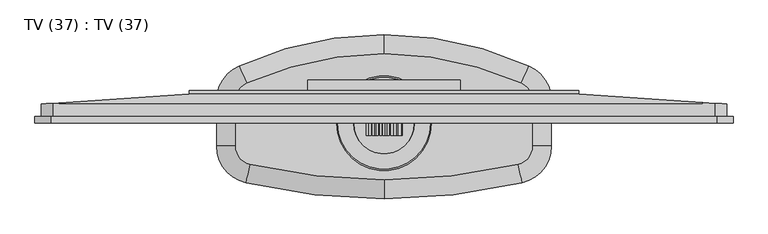
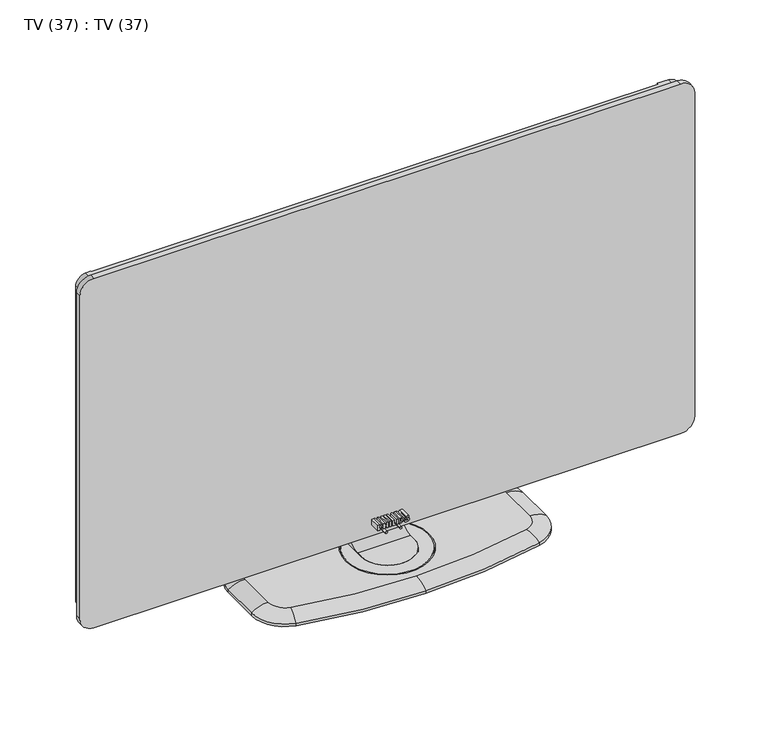
"""IFC4 building model written with IfcOpenShell, lengths in millimetres: furniture geometry, TV (37) : TV (37)."""

import ifcopenshell
import ifcopenshell.guid

model = None  # the IFC model being written
_history = None  # IfcOwnerHistory: only IFC2X3 demands one
_inside = {}  # id of a spatial element -> (the spatial element, [elements in it])
_under = {}  # id of a project, library or spatial element -> (it, [spatial elements below it])
_declared = {}  # id of a project -> (the project, [libraries it declares])
_typed = {}  # id of a type object -> (the type object, [elements of that type])
_made_of = {}  # id of a material, layer set ... -> (it, [elements and type objects made of it])


def new_model(schema):
    """Start an empty IFC model of exactly this schema.

    Asked for "IFC4X3", IfcOpenShell would pick the latest addendum, in which some entities
    have other attributes; the version numbers below select the first issue.
    IFC2X3 requires an IfcOwnerHistory on every rooted entity: one is made here for all.
    """
    global model, _history
    if schema == "IFC4X3":
        model = ifcopenshell.file(schema_version=(4, 3, 0, 0))
    else:
        model = ifcopenshell.file(schema=schema)
    _inside.clear()
    _under.clear()
    _declared.clear()
    _typed.clear()
    _made_of.clear()
    _history = None
    if model.schema == "IFC2X3":
        org = make("IfcOrganization", Name="unknown")
        user = make(
            "IfcPersonAndOrganization",
            ThePerson=make("IfcPerson", FamilyName="unknown"),
            TheOrganization=org,
        )
        app = make(
            "IfcApplication",
            ApplicationDeveloper=org,
            Version="unknown",
            ApplicationFullName="unknown",
            ApplicationIdentifier="unknown",
        )
        _history = make(
            "IfcOwnerHistory",
            OwningUser=user,
            OwningApplication=app,
            ChangeAction="ADDED",
            CreationDate=0,
        )
    return model


def make(cls, **values):
    """One entity of the class cls with the attributes given. An attribute that is None is left unset."""
    return model.create_entity(
        cls, **{name: value for name, value in values.items() if value is not None}
    )


def rooted(cls, **values):
    """An entity with a GlobalId (a new one), such as an element, a storey or a relation."""
    return make(cls, GlobalId=ifcopenshell.guid.new(), OwnerHistory=_history, **values)


def si_unit(unit_type, name, prefix=None):
    """IfcSIUnit, for example si_unit("LENGTHUNIT", "METRE", prefix="MILLI")."""
    return make("IfcSIUnit", UnitType=unit_type, Prefix=prefix, Name=name)


def assignment(units):
    """IfcUnitAssignment: the units of a project."""
    return None if units is None else make("IfcUnitAssignment", Units=units)


def point(xyz):
    """IfcCartesianPoint."""
    return None if xyz is None else make("IfcCartesianPoint", Coordinates=xyz)


def direction(xyz):
    """IfcDirection."""
    return None if xyz is None else make("IfcDirection", DirectionRatios=xyz)


def frame(location, z_axis=None, x_axis=None):
    """IfcAxis2Placement3D, a coordinate frame: its origin and axes. An axis left out is left unset."""
    return make(
        "IfcAxis2Placement3D",
        Location=point(location),
        Axis=direction(z_axis),
        RefDirection=direction(x_axis),
    )


def frame_2d(location, x_axis=None):
    """IfcAxis2Placement2D, a coordinate frame in the plane: its origin and x axis."""
    return make(
        "IfcAxis2Placement2D", Location=point(location), RefDirection=direction(x_axis)
    )


def origin():
    """The frame at (0, 0, 0) with its axes left unset."""
    return frame((0.0, 0.0, 0.0))


def place(relative_to, where):
    """IfcLocalPlacement: puts the frame where relative to a parent placement (None: the world)."""
    return make(
        "IfcLocalPlacement", PlacementRelTo=relative_to, RelativePlacement=where
    )


def context(
    kind, dimensions, precision=None, world=None, true_north=None, identifier=None
):
    """IfcGeometricRepresentationContext, for example the 3D "Model" context."""
    return make(
        "IfcGeometricRepresentationContext",
        ContextIdentifier=identifier,
        ContextType=kind,
        CoordinateSpaceDimension=dimensions,
        Precision=precision,
        WorldCoordinateSystem=world,
        TrueNorth=true_north,
    )


def project(units=None, contexts=None):
    """IfcProject with its units and contexts."""
    return rooted(
        "IfcProject",
        Name="project",
        RepresentationContexts=contexts,
        UnitsInContext=assignment(units),
    )


def spatial(cls, under=None, at=None, **own):
    """A site, building, storey or space (cls), placed at a placement, below another one or the project."""
    s = rooted(cls, ObjectPlacement=at, **own)
    if under is not None:
        _under.setdefault(under.id(), (under, []))[1].append(s)
    return s


def polyline(points):
    """IfcPolyline through the points."""
    return make("IfcPolyline", Points=[point(p) for p in points])


def circle_curve(where, radius):
    """IfcCircle in the frame where."""
    return make("IfcCircle", Position=where, Radius=radius)


def ellipse_curve(where, semi_axis1, semi_axis2):
    """IfcEllipse in the frame where."""
    return make(
        "IfcEllipse", Position=where, SemiAxis1=semi_axis1, SemiAxis2=semi_axis2
    )


def trimmed(basis, trim1, trim2, sense, master):
    """IfcTrimmedCurve: the piece of a basis curve between two trims."""
    return make(
        "IfcTrimmedCurve",
        BasisCurve=basis,
        Trim1=trim1,
        Trim2=trim2,
        SenseAgreement=sense,
        MasterRepresentation=master,
    )


def segment(curve, same_sense, transition):
    """IfcCompositeCurveSegment."""
    return make(
        "IfcCompositeCurveSegment",
        Transition=transition,
        SameSense=same_sense,
        ParentCurve=curve,
    )


def composite_curve(segments, self_intersect=None):
    """IfcCompositeCurve: segments joined end to end."""
    return make("IfcCompositeCurve", Segments=segments, SelfIntersect=self_intersect)


def outline(outer, holes=None, kind="AREA"):
    """IfcArbitraryClosedProfileDef: a profile drawn as a closed curve; with holes, ...WithVoids."""
    if holes is None:
        return make("IfcArbitraryClosedProfileDef", ProfileType=kind, OuterCurve=outer)
    return make(
        "IfcArbitraryProfileDefWithVoids",
        ProfileType=kind,
        OuterCurve=outer,
        InnerCurves=holes,
    )


def extrude(swept, where, along, depth):
    """IfcExtrudedAreaSolid: the profile swept, set in the frame where, extruded along a direction by depth."""
    return make(
        "IfcExtrudedAreaSolid",
        SweptArea=swept,
        Position=where,
        ExtrudedDirection=direction(along),
        Depth=depth,
    )


def shape(context_of_items, identifier, shape_type, items):
    """IfcShapeRepresentation: the items that make up one representation, for example the "Body"."""
    return make(
        "IfcShapeRepresentation",
        ContextOfItems=context_of_items,
        RepresentationIdentifier=identifier,
        RepresentationType=shape_type,
        Items=items,
    )


def source(mapping_origin, context_of_items, identifier, shape_type, items):
    """IfcRepresentationMap: a shape defined once, which mapped items show again and again."""
    return make(
        "IfcRepresentationMap",
        MappingOrigin=mapping_origin,
        MappedRepresentation=shape(context_of_items, identifier, shape_type, items),
    )


def transform(
    local_origin,
    x_axis=None,
    y_axis=None,
    z_axis=None,
    scale=None,
    scale2=None,
    scale3=None,
    uniform=True,
):
    """IfcCartesianTransformationOperator3D, or its non-uniform kind. x_axis, y_axis, z_axis: its Axis1, 2, 3."""
    if uniform:
        return make(
            "IfcCartesianTransformationOperator3D",
            Axis1=direction(x_axis),
            Axis2=direction(y_axis),
            LocalOrigin=point(local_origin),
            Scale=scale,
            Axis3=direction(z_axis),
        )
    return make(
        "IfcCartesianTransformationOperator3DnonUniform",
        Axis1=direction(x_axis),
        Axis2=direction(y_axis),
        LocalOrigin=point(local_origin),
        Scale=scale,
        Axis3=direction(z_axis),
        Scale2=scale2,
        Scale3=scale3,
    )


def mapped(mapping_source, mapping_target):
    """IfcMappedItem: shows the shape of a source again, moved by a transform."""
    return make(
        "IfcMappedItem", MappingSource=mapping_source, MappingTarget=mapping_target
    )


def made_of(thing, what):
    """Note that an element or type object is made of a material, layer set ...; save() writes the relation."""
    if what is not None:
        _made_of.setdefault(what.id(), (what, []))[1].append(thing)
    return thing


def element(
    cls,
    number,
    at=None,
    inside=None,
    cuts=None,
    type_object=None,
    material=None,
    context=None,
    identifier="Body",
    shape_type=None,
    held_by="IfcProductDefinitionShape",
    body=None,
    shapes=None,
    **own,
):
    """One element of the class cls, such as IfcWall. Its Tag is "e" and its number.

    at: its placement. inside: the storey or other place that contains it. cuts: it is an
    opening in that element (IfcRelVoidsElement). A single representation is given by context,
    identifier, shape_type and body (its items); several are given by shapes. held_by: the class
    of the entity that holds the representations. save() writes the other relations.
    """
    e = rooted(cls, Tag="e%d" % number, ObjectPlacement=at, **own)
    if body is not None:
        shapes = [shape(context, identifier, shape_type, body)]
    if shapes is not None:
        e.Representation = make(held_by, Representations=shapes)
    if inside is not None:
        _inside.setdefault(inside.id(), (inside, []))[1].append(e)
    if cuts is not None:
        rooted(
            "IfcRelVoidsElement", RelatingBuildingElement=cuts, RelatedOpeningElement=e
        )
    if type_object is not None:
        _typed.setdefault(type_object.id(), (type_object, []))[1].append(e)
    return made_of(e, material)


def aggregate(whole, parts):
    """IfcRelAggregates: a whole, such as a stair, and the parts it consists of."""
    return rooted("IfcRelAggregates", RelatingObject=whole, RelatedObjects=parts)


def save(model, path):
    """Write the relations noted so far, then the file.

    IfcRelAggregates (storeys below a building ...), IfcRelContainedInSpatialStructure (elements
    in a storey), IfcRelDefinesByType, IfcRelAssociatesMaterial and IfcRelDeclares: one each for
    every whole, place, type object, material and project.
    """
    for whole, parts in _under.values():
        aggregate(whole, parts)
    for where, things in _inside.values():
        rooted(
            "IfcRelContainedInSpatialStructure",
            RelatedElements=things,
            RelatingStructure=where,
        )
    for kind, things in _typed.values():
        rooted("IfcRelDefinesByType", RelatedObjects=things, RelatingType=kind)
    for what, things in _made_of.values():
        rooted("IfcRelAssociatesMaterial", RelatedObjects=things, RelatingMaterial=what)
    for by, libraries in _declared.values():
        rooted("IfcRelDeclares", RelatingContext=by, RelatedDefinitions=libraries)
    model.write(path)


def plane_surface(at):
    """IfcPlane: the flat surface through the origin of the frame at, square to its z axis."""
    return make("IfcPlane", Position=at)


def cylinder_surface(at, radius):
    """IfcCylindricalSurface: all points at the distance radius from the z axis of the frame at."""
    return make("IfcCylindricalSurface", Position=at, Radius=radius)


def revolved_surface(curve, axis_point, axis_direction):
    """IfcSurfaceOfRevolution: the curve turned about the line through axis_point along axis_direction."""
    return make(
        "IfcSurfaceOfRevolution",
        SweptCurve=make("IfcArbitraryOpenProfileDef", ProfileType="CURVE", Curve=curve),
        AxisPosition=make("IfcAxis1Placement", Location=point(axis_point), Axis=direction(axis_direction)),
    )


def advanced_brep(points, edges, surfaces, faces):
    """IfcAdvancedBrep: a solid bounded by faces that lie on surfaces and meet in shared edges.

    An edge is (start, end): straight between two places in points (the first is 0);
    or (start, end, curve); or (start, end, curve, False) where it runs against its curve.
    A face is (place in surfaces, loops), or (place, loops, False) where it looks against
    its surface's normal. A loop lists edges by number (the first is 1), with a minus sign
    where the edge is run from its end to its start. The first loop is the outer one.
    """
    corners = [point(p) for p in points]
    vertices = [make("IfcVertexPoint", VertexGeometry=c) for c in corners]
    made = []
    for start, end, *more in edges:
        made.append(
            make(
                "IfcEdgeCurve",
                EdgeStart=vertices[start],
                EdgeEnd=vertices[end],
                EdgeGeometry=more[0] if more else make("IfcPolyline", Points=[corners[start], corners[end]]),
                SameSense=more[1] if len(more) > 1 else True,
            )
        )
    hull = []
    for where, loops, *sense in faces:
        bounds = []
        for j, loop in enumerate(loops):
            ring = [make("IfcOrientedEdge", EdgeElement=made[abs(k) - 1], Orientation=k > 0) for k in loop]
            bounds.append(
                make(
                    "IfcFaceOuterBound" if j == 0 else "IfcFaceBound",
                    Bound=make("IfcEdgeLoop", EdgeList=ring),
                    Orientation=True,
                )
            )
        hull.append(make("IfcAdvancedFace", Bounds=bounds, FaceSurface=surfaces[where], SameSense=sense[0] if sense else True))
    return make("IfcAdvancedBrep", Outer=make("IfcClosedShell", CfsFaces=hull))


def tv_37_tv_37_058471c0(model_context):
    return source(origin(), model_context, "Body", "SolidModel", [
        advanced_brep(
        [(47.5, 88.0, 133.1843541), (47.5, 88.0, 218.1843541), (47.5, 78.0, 218.1843541), (47.5, 78.0, 133.6678583), (47.5, 59.7827761, 41.2895959), (47.5, 32.0312094, 20.0814552), (47.5, 29.7558767, 20.0), (47.5, 18.8623336, 20.0), (47.5, 18.8623336, 10.0), (47.5, 44.5, 10.0), (47.5, 69.2193203, 37.9802704), (-47.5, 88.0, 133.1843541), (-47.5, 69.2193203, 37.9802704), (-47.5, 44.5, 10.0), (-47.5, 18.8623336, 10.0), (-47.5, 18.8623336, 20.0), (-47.5, 29.7558767, 20.0), (-47.5, 32.0312094, 20.0814552), (-47.5, 59.7827761, 41.2895959), (-47.5, 78.0, 133.6678583), (-47.5, 78.0, 218.1843541), (-47.5, 88.0, 218.1843541)],
        [
            (0, 1),
            (1, 2),
            (2, 3),
            (3, 4, circle_curve(frame((47.5, -252.8458142, 150.9261062), z_axis=(-1.0, 0.0, 0.0), x_axis=(0.0, 1.0, 0.0)), 331.2956382)),
            (4, 5, circle_curve(frame((47.5, 29.7558767, 51.8198052), z_axis=(-1.0, 0.0, 0.0), x_axis=(0.0, 1.0, 0.0)), 31.8198052)),
            (5, 6, circle_curve(frame((47.5, 29.7558767, 51.8198052), z_axis=(-1.0, 0.0, 0.0), x_axis=(0.0, 1.0, 0.0)), 31.8198052)),
            (6, 7),
            (7, 8),
            (8, 9),
            (9, 10, circle_curve(frame((47.5, 16.5507824, 59.6012298), z_axis=(1.0, 0.0, 0.0), x_axis=(0.0, 1.0, 0.0)), 56.9336523)),
            (10, 0, circle_curve(frame((47.5, -162.6973021, 133.1843541), z_axis=(1.0, 0.0, 0.0), x_axis=(0.0, 1.0, 0.0)), 250.6973021)),
            (11, 12, circle_curve(frame((-47.5, -162.6973021, 133.1843541), z_axis=(-1.0, 0.0, 0.0), x_axis=(0.0, 1.0, 0.0)), 250.6973021)),
            (12, 13, circle_curve(frame((-47.5, 16.5507824, 59.6012298), z_axis=(-1.0, 0.0, 0.0), x_axis=(0.0, 1.0, 0.0)), 56.9336523)),
            (13, 14),
            (14, 15),
            (15, 16),
            (16, 17, circle_curve(frame((-47.5, 29.7558767, 51.8198052), z_axis=(1.0, 0.0, 0.0), x_axis=(0.0, 1.0, 0.0)), 31.8198052)),
            (17, 18, circle_curve(frame((-47.5, 29.7558767, 51.8198052), z_axis=(1.0, 0.0, 0.0), x_axis=(0.0, 1.0, 0.0)), 31.8198052)),
            (18, 19, circle_curve(frame((-47.5, -252.8458142, 150.9261062), z_axis=(1.0, 0.0, 0.0), x_axis=(0.0, 1.0, 0.0)), 331.2956382)),
            (19, 20),
            (20, 21),
            (21, 11),
            (0, 11),
            (21, 1),
            (20, 2),
            (19, 3),
            (18, 4),
            (16, 6),
            (15, 7, circle_curve(frame((0.0, 18.8623336, 20.0), z_axis=(0.0, 0.0, 1.0), x_axis=(1.0, 0.0, 0.0)), 47.5)),
            (8, 14, circle_curve(frame((0.0, 18.8623336, 10.0), z_axis=(0.0, 0.0, -1.0), x_axis=(1.0, 0.0, 0.0)), 47.5)),
            (13, 9),
            (12, 10),
        ],
        [
            plane_surface(frame((47.5, 88.0, 393.1843541), z_axis=(1.0, 0.0, 0.0), x_axis=(0.0, 0.0, 1.0))),
            plane_surface(frame((-47.5, 88.0, 393.1843541), z_axis=(-1.0, 0.0, 0.0), x_axis=(0.0, 0.0, -1.0))),
            plane_surface(frame((47.5, 88.0, 133.1843541), z_axis=(0.0, 1.0, 0.0), x_axis=(-1.0, 0.0, 0.0))),
            plane_surface(frame((47.5, 88.0, 218.1843541), z_axis=(0.0, 0.0, 1.0), x_axis=(-1.0, 0.0, 0.0))),
            plane_surface(frame((47.5, 78.0, 218.1843541), z_axis=(0.0, -1.0, 0.0), x_axis=(-1.0, 0.0, 0.0))),
            revolved_surface(polyline([(-47.5, 78.44982399999998, 150.9261062), (47.5, 78.44982399999998, 150.9261062)]), (-47.5, -252.8458142, 150.9261062), (-1.0, 0.0, 0.0)),
            revolved_surface(polyline([(-47.5, 61.575681900000006, 51.8198052), (47.5, 61.575681900000006, 51.8198052)]), (-47.5, 29.7558767, 51.8198052), (-1.0, 0.0, 0.0)),
            plane_surface(frame((47.5, 29.7558767, 20.0), z_axis=(0.0, 0.0, 1.0), x_axis=(-1.0, 0.0, 0.0))),
            plane_surface(frame((47.5, 18.8623336, 10.0), z_axis=(0.0, 0.0, -1.0), x_axis=(-1.0, 0.0, 0.0))),
            cylinder_surface(frame((-47.5, 16.5507824, 59.6012298), z_axis=(1.0, 0.0, 0.0), x_axis=(0.0, 1.0, 0.0)), 56.9336523),
            cylinder_surface(frame((-47.5, -162.6973021, 133.1843541), z_axis=(1.0, 0.0, 0.0), x_axis=(0.0, 1.0, 0.0)), 250.6973021),
            cylinder_surface(frame((0.0, 18.8623336, 10.0), z_axis=(0.0, 0.0, 1.0), x_axis=(1.0, 0.0, 0.0)), 47.5),
        ],
        [
            (0, [[1, 2, 3, 4, 5, 6, 7, 8, 9, 10, 11]]),
            (1, [[12, 13, 14, 15, 16, 17, 18, 19, 20, 21, 22]]),
            (2, [[-1, 23, -22, 24]]),
            (3, [[-2, -24, -21, 25]]),
            (4, [[-3, -25, -20, 26]]),
            (5, [[-4, -26, -19, 27]]),
            (6, [[-27, -18, -17, 28, -6, -5]]),
            (7, [[-7, -28, -16, 29]]),
            (8, [[30, -14, 31, -9]]),
            (9, [[-10, -31, -13, 32]]),
            (10, [[-11, -32, -12, -23]]),
            (11, [[-29, -15, -30, -8]]),
        ],
    ),
        advanced_brep(
        [(-205.0, 88.7099995, 0.0), (-205.0, -47.2603519, 0.0), (-205.0, -47.2603519, 5.0), (-205.0, 88.7099995, 5.0), (-218.5849057, -74.9290034, 5.0), (-265.0, -16.4871491, 5.0), (-265.0, 55.9989024, 5.0), (-229.622384, 110.7139662, 5.0), (0.0, 160.0, 5.0), (229.622384, 110.7139662, 5.0), (265.0, 55.9989024, 5.0), (265.0, -16.4871491, 5.0), (218.5849057, -74.9290034, 5.0), (0.0, -100.0, 5.0), (0.0, -70.0, 5.0), (205.0, -47.2603519, 5.0), (205.0, 88.7099995, 5.0), (0.0, 130.0, 5.0), (-211.7924528, -45.7080763, 20.0), (0.0, -70.0, 20.0), (211.7924528, -45.7080763, 20.0), (235.0, -16.4871491, 20.0), (235.0, 55.9989024, 20.0), (217.311192, 83.3564343, 20.0), (0.0, 130.0, 20.0), (-217.311192, 83.3564343, 20.0), (-235.0, 55.9989024, 20.0), (-235.0, -16.4871491, 20.0), (75.0, 19.7558767, 20.0), (-75.0, 19.7558767, 20.0), (73.0, 19.7558767, 20.0), (-73.0, 19.7558767, 20.0), (48.0, 19.7558767, 20.0), (-48.0, 19.7558767, 20.0), (-48.0, 59.7558767, 20.0), (48.0, 59.7558767, 20.0), (205.0, -47.2603519, 0.0), (205.0, 88.7099995, 0.0), (0.0, 130.0, 0.0), (0.0, -70.0, 0.0), (-218.5849057, -74.9290034, 10.0), (0.0, -100.0, 10.0), (-265.0, -16.4871491, 10.0), (-265.0, 55.9989024, 10.0), (-229.622384, 110.7139662, 10.0), (0.0, 160.0, 10.0), (218.5849057, -74.9290034, 10.0), (265.0, -16.4871491, 10.0), (265.0, 55.9989024, 10.0), (229.622384, 110.7139662, 10.0), (-75.0, 19.7558767, 10.0), (75.0, 19.7558767, 10.0), (-73.0, 19.7558767, 10.0), (73.0, 19.7558767, 10.0), (48.0, 19.7558767, 10.0), (48.0, 59.7558767, 10.0), (-48.0, 59.7558767, 10.0), (-48.0, 19.7558767, 10.0)],
        [
            (0, 1),
            (1, 2),
            (2, 3),
            (3, 0),
            (4, 5, circle_curve(frame((-205.0, -16.4871491, 5.0), z_axis=(0.0, 0.0, -1.0), x_axis=(-0.22641509433980192, -0.9740309055954531, 0.0)), 60.0)),
            (5, 6),
            (6, 7, circle_curve(frame((-205.0, 55.9989024, 5.0), z_axis=(0.0, 0.0, -1.0), x_axis=(-1.0, 0.0, 0.0)), 60.0)),
            (7, 8, circle_curve(frame((0.0, -399.5454545, 5.0), z_axis=(0.0, 0.0, -1.0), x_axis=(-0.41037306642402943, 0.911917730035851, 0.0)), 559.5454545)),
            (8, 9, circle_curve(frame((0.0, -399.5454545, 5.0), z_axis=(0.0, 0.0, -1.0), x_axis=(0.41037306642402943, 0.911917730035851, 0.0)), 559.5454545)),
            (9, 10, circle_curve(frame((205.0, 55.9989024, 5.0), z_axis=(0.0, 0.0, -1.0), x_axis=(1.0, 0.0, 0.0)), 60.0)),
            (10, 11),
            (11, 12, circle_curve(frame((205.0, -16.4871491, 5.0), z_axis=(0.0, 0.0, -1.0), x_axis=(0.22641509433980192, -0.9740309055954531, 0.0)), 60.0)),
            (12, 13, circle_curve(frame((0.0, 865.4166667, 5.0), z_axis=(0.0, 0.0, -1.0), x_axis=(0.0, -1.0, 0.0)), 965.4166667)),
            (13, 4, circle_curve(frame((0.0, 865.4166667, 5.0), z_axis=(0.0, 0.0, -1.0), x_axis=(0.0, -1.0, 0.0)), 965.4166667)),
            (2, 14, circle_curve(frame((0.0, 865.4166667, 5.0), z_axis=(0.0, 0.0, 1.0), x_axis=(0.0, -1.0, 0.0)), 935.4166667)),
            (14, 15, circle_curve(frame((0.0, 865.4166667, 5.0), z_axis=(0.0, 0.0, 1.0), x_axis=(0.0, -1.0, 0.0)), 935.4166667)),
            (15, 16),
            (16, 17, circle_curve(frame((0.0, -399.5454545, 5.0), z_axis=(0.0, 0.0, 1.0), x_axis=(0.41037306642402943, 0.911917730035851, 0.0)), 529.5454545)),
            (17, 3, circle_curve(frame((0.0, -399.5454545, 5.0), z_axis=(0.0, 0.0, 1.0), x_axis=(-0.41037306642402943, 0.911917730035851, 0.0)), 529.5454545)),
            (18, 19, circle_curve(frame((0.0, 865.4166667, 20.0), z_axis=(0.0, 0.0, 1.0), x_axis=(0.0, -1.0, 0.0)), 935.4166667)),
            (19, 20, circle_curve(frame((0.0, 865.4166667, 20.0), z_axis=(0.0, 0.0, 1.0), x_axis=(0.0, -1.0, 0.0)), 935.4166667)),
            (20, 21, circle_curve(frame((205.0, -16.4871491, 20.0), z_axis=(0.0, 0.0, 1.0), x_axis=(0.22641509433980192, -0.9740309055954531, 0.0)), 30.0)),
            (21, 22),
            (22, 23, circle_curve(frame((205.0, 55.9989024, 20.0), z_axis=(0.0, 0.0, 1.0), x_axis=(1.0, 0.0, 0.0)), 30.0)),
            (23, 24, circle_curve(frame((0.0, -399.5454545, 20.0), z_axis=(0.0, 0.0, 1.0), x_axis=(0.41037306642402943, 0.911917730035851, 0.0)), 529.5454545)),
            (24, 25, circle_curve(frame((0.0, -399.5454545, 20.0), z_axis=(0.0, 0.0, 1.0), x_axis=(-0.41037306642402943, 0.911917730035851, 0.0)), 529.5454545)),
            (25, 26, circle_curve(frame((-205.0, 55.9989024, 20.0), z_axis=(0.0, 0.0, 1.0), x_axis=(-1.0, 0.0, 0.0)), 30.0)),
            (26, 27),
            (27, 18, circle_curve(frame((-205.0, -16.4871491, 20.0), z_axis=(0.0, 0.0, 1.0), x_axis=(-0.22641509433980192, -0.9740309055954531, 0.0)), 30.0)),
            (28, 29, circle_curve(frame((0.0, 19.7558767, 20.0), z_axis=(0.0, 0.0, -1.0), x_axis=(1.0, 0.0, 0.0)), 75.0)),
            (29, 28, circle_curve(frame((0.0, 19.7558767, 20.0), z_axis=(0.0, 0.0, -1.0), x_axis=(1.0, 0.0, 0.0)), 75.0)),
            (30, 31, circle_curve(frame((0.0, 19.7558767, 20.0), z_axis=(0.0, 0.0, 1.0), x_axis=(1.0, 0.0, 0.0)), 73.0)),
            (31, 30, circle_curve(frame((0.0, 19.7558767, 20.0), z_axis=(0.0, 0.0, 1.0), x_axis=(1.0, 0.0, 0.0)), 73.0)),
            (32, 33, circle_curve(frame((0.0, 19.7558767, 20.0), z_axis=(0.0, 0.0, -1.0), x_axis=(1.0, 0.0, 0.0)), 48.0)),
            (33, 34),
            (34, 35),
            (35, 32),
            (15, 36),
            (36, 37),
            (37, 16),
            (0, 38, circle_curve(frame((0.0, -399.5454545, 0.0), z_axis=(0.0, 0.0, -1.0), x_axis=(-0.41037306642402943, 0.911917730035851, 0.0)), 529.5454545)),
            (38, 37, circle_curve(frame((0.0, -399.5454545, 0.0), z_axis=(0.0, 0.0, -1.0), x_axis=(0.41037306642402943, 0.911917730035851, 0.0)), 529.5454545)),
            (36, 39, circle_curve(frame((0.0, 865.4166667, 0.0), z_axis=(0.0, 0.0, -1.0), x_axis=(0.0, -1.0, 0.0)), 935.4166667)),
            (39, 1, circle_curve(frame((0.0, 865.4166667, 0.0), z_axis=(0.0, 0.0, -1.0), x_axis=(0.0, -1.0, 0.0)), 935.4166667)),
            (18, 40, circle_curve(frame((-211.7924528, -45.7080763, -30.0), z_axis=(0.9740309055954945, -0.22641509433962398, 0.0), x_axis=(0.22641509433962398, 0.9740309055954945, 0.0)), 50.0)),
            (40, 41, circle_curve(frame((0.0, 865.4166667, 10.0), z_axis=(0.0, 0.0, 1.0), x_axis=(0.0, -1.0, 0.0)), 965.4166667)),
            (41, 19, circle_curve(frame((0.0, -70.0, -30.0), z_axis=(-1.0, 0.0, 0.0), x_axis=(0.0, 1.0, 0.0)), 50.0)),
            (39, 14),
            (40, 4),
            (13, 41),
            (27, 42, circle_curve(frame((-235.0, -16.4871491, -30.0), z_axis=(0.0, -1.0, 0.0), x_axis=(1.0, 0.0, 0.0)), 50.0)),
            (42, 40, circle_curve(frame((-205.0, -16.4871491, 10.0), z_axis=(0.0, 0.0, 1.0), x_axis=(-0.22641509433980192, -0.9740309055954531, 0.0)), 60.0)),
            (42, 5),
            (26, 43, circle_curve(frame((-235.0, 55.9989024, -30.0), z_axis=(0.0, -1.0, 0.0), x_axis=(1.0, 0.0, 0.0)), 50.0)),
            (43, 42),
            (43, 6),
            (25, 44, circle_curve(frame((-217.311192, 83.3564343, -30.0), z_axis=(-0.9119177300358057, -0.41037306642413024, 0.0), x_axis=(0.41037306642413024, -0.9119177300358057, 0.0)), 50.0)),
            (44, 43, circle_curve(frame((-205.0, 55.9989024, 10.0), z_axis=(0.0, 0.0, 1.0), x_axis=(-1.0, 0.0, 0.0)), 60.0)),
            (44, 7),
            (24, 45, circle_curve(frame((0.0, 130.0, -30.0), z_axis=(-1.0, 0.0, 0.0), x_axis=(0.0, -1.0, 0.0)), 50.0)),
            (45, 44, circle_curve(frame((0.0, -399.5454545, 10.0), z_axis=(0.0, 0.0, 1.0), x_axis=(-0.41037306642402943, 0.911917730035851, 0.0)), 559.5454545)),
            (17, 38),
            (45, 8),
            (12, 46),
            (46, 41, circle_curve(frame((0.0, 865.4166667, 10.0), z_axis=(0.0, 0.0, -1.0), x_axis=(0.0, -1.0, 0.0)), 965.4166667)),
            (46, 20, circle_curve(frame((211.7924528, -45.7080763, -30.0), z_axis=(-0.9740309055954932, -0.2264150943396295, 0.0), x_axis=(-0.2264150943396295, 0.9740309055954932, 0.0)), 50.0)),
            (11, 47),
            (47, 46, circle_curve(frame((205.0, -16.4871491, 10.0), z_axis=(0.0, 0.0, -1.0), x_axis=(0.22641509433980192, -0.9740309055954531, 0.0)), 60.0)),
            (47, 21, circle_curve(frame((235.0, -16.4871491, -30.0), z_axis=(0.0, -1.0, 0.0), x_axis=(-1.0, 0.0, 0.0)), 50.0)),
            (10, 48),
            (48, 47),
            (48, 22, circle_curve(frame((235.0, 55.9989024, -30.0), z_axis=(0.0, -1.0, 0.0), x_axis=(-1.0, 0.0, 0.0)), 50.0)),
            (9, 49),
            (49, 48, circle_curve(frame((205.0, 55.9989024, 10.0), z_axis=(0.0, 0.0, -1.0), x_axis=(1.0, 0.0, 0.0)), 60.0)),
            (49, 23, circle_curve(frame((217.311192, 83.3564343, -30.0), z_axis=(0.9119177300358283, -0.41037306642407984, 0.0), x_axis=(-0.41037306642407984, -0.9119177300358283, 0.0)), 50.0)),
            (45, 49, circle_curve(frame((0.0, -399.5454545, 10.0), z_axis=(0.0, 0.0, -1.0), x_axis=(0.41037306642402943, 0.911917730035851, 0.0)), 559.5454545)),
            (50, 51, circle_curve(frame((0.0, 19.7558767, 10.0), z_axis=(0.0, 0.0, 1.0), x_axis=(1.0, 0.0, 0.0)), 75.0)),
            (51, 50, circle_curve(frame((0.0, 19.7558767, 10.0), z_axis=(0.0, 0.0, 1.0), x_axis=(1.0, 0.0, 0.0)), 75.0)),
            (52, 53, circle_curve(frame((0.0, 19.7558767, 10.0), z_axis=(0.0, 0.0, -1.0), x_axis=(1.0, 0.0, 0.0)), 73.0)),
            (53, 52, circle_curve(frame((0.0, 19.7558767, 10.0), z_axis=(0.0, 0.0, -1.0), x_axis=(1.0, 0.0, 0.0)), 73.0)),
            (54, 55),
            (55, 56),
            (56, 57),
            (57, 54, circle_curve(frame((0.0, 19.7558767, 10.0), z_axis=(0.0, 0.0, 1.0), x_axis=(1.0, 0.0, 0.0)), 48.0)),
            (50, 29),
            (28, 51),
            (52, 31),
            (30, 53),
            (54, 32),
            (35, 55),
            (34, 56),
            (33, 57),
        ],
        [
            plane_surface(frame((-205.0, 190.0, 0.0), z_axis=(-1.0, 0.0, 0.0), x_axis=(0.0, -1.0, 0.0))),
            plane_surface(frame((-205.0, 190.0, 5.0), z_axis=(0.0, 0.0, -1.0), x_axis=(0.0, -1.0, 0.0))),
            plane_surface(frame((-295.0, 190.0, 20.0), z_axis=(0.0, 0.0, 1.0), x_axis=(0.0, -1.0, 0.0))),
            plane_surface(frame((205.0, 190.0, 5.0), z_axis=(1.0, 0.0, 0.0), x_axis=(0.0, -1.0, 0.0))),
            plane_surface(frame((205.0, 190.0, 0.0), z_axis=(0.0, 0.0, -1.0), x_axis=(0.0, -1.0, 0.0))),
            revolved_surface(trimmed(ellipse_curve(frame((0.0, -70.0, -30.0), z_axis=(1.0, 0.0, 0.0), x_axis=(0.0, 1.0, 0.0)), 50.0, 50.0), [point((0.0, -70.0, 20.0))], [point((0.0, -100.0, 10.0))], True, "CARTESIAN"), (0.0, 865.4166667, 0.0), (0.0, 0.0, -1.0)),
            cylinder_surface(frame((0.0, 865.4166667, 0.0), z_axis=(0.0, 0.0, -1.0), x_axis=(0.0, -1.0, 0.0)), 935.4166667),
            cylinder_surface(frame((0.0, 865.4166667, 0.0), z_axis=(0.0, 0.0, -1.0), x_axis=(0.0, -1.0, 0.0)), 965.4166667),
            revolved_surface(trimmed(ellipse_curve(frame((-211.7924528, -45.7080763, -30.0), z_axis=(0.9740309055954531, -0.22641509433980195, 0.0), x_axis=(0.22641509433980195, 0.9740309055954531, 0.0)), 50.0, 50.0), [point((-211.7924528, -45.7080763, 20.0))], [point((-218.5849057, -74.9290034, 10.0))], True, "CARTESIAN"), (-205.0, -16.4871491, 0.0), (0.0, 0.0, -1.0)),
            cylinder_surface(frame((-205.0, -16.4871491, 0.0), z_axis=(0.0, 0.0, -1.0), x_axis=(-0.22641509433980192, -0.9740309055954531, 0.0)), 60.0),
            cylinder_surface(frame((-235.0, -16.4871491, -30.0), z_axis=(0.0, 1.0, 0.0), x_axis=(1.0, 0.0, 0.0)), 50.0),
            plane_surface(frame((-265.0, -16.4871491, 5.0), z_axis=(-1.0, 0.0, 0.0), x_axis=(0.0, 1.0, 0.0))),
            revolved_surface(trimmed(ellipse_curve(frame((-235.0, 55.9989024, -30.0), z_axis=(0.0, -1.0, 0.0), x_axis=(1.0, 0.0, 0.0)), 50.0, 50.0), [point((-235.0, 55.9989024, 20.0))], [point((-265.0, 55.9989024, 10.0))], True, "CARTESIAN"), (-205.0, 55.9989024, 0.0), (0.0, 0.0, -1.0)),
            cylinder_surface(frame((-205.0, 55.9989024, 0.0), z_axis=(0.0, 0.0, -1.0), x_axis=(-1.0, 0.0, 0.0)), 60.0),
            revolved_surface(trimmed(ellipse_curve(frame((-217.311192, 83.3564343, -30.0), z_axis=(-0.911917730035851, -0.41037306642402943, 0.0), x_axis=(0.41037306642402943, -0.911917730035851, 0.0)), 50.0, 50.0), [point((-217.311192, 83.3564343, 20.0))], [point((-229.622384, 110.7139662, 10.0))], True, "CARTESIAN"), (0.0, -399.5454545, 0.0), (0.0, 0.0, -1.0)),
            cylinder_surface(frame((0.0, -399.5454545, 0.0), z_axis=(0.0, 0.0, -1.0), x_axis=(-0.41037306642402943, 0.911917730035851, 0.0)), 529.5454545),
            cylinder_surface(frame((0.0, -399.5454545, 0.0), z_axis=(0.0, 0.0, -1.0), x_axis=(-0.41037306642402943, 0.911917730035851, 0.0)), 559.5454545),
            cylinder_surface(frame((0.0, 865.4166667, 0.0), z_axis=(0.0, 0.0, 1.0), x_axis=(0.0, -1.0, 0.0)), 965.4166667),
            cylinder_surface(frame((0.0, 865.4166667, 0.0), z_axis=(0.0, 0.0, 1.0), x_axis=(0.0, -1.0, 0.0)), 935.4166667),
            revolved_surface(trimmed(ellipse_curve(frame((0.0, -70.0, -30.0), z_axis=(-1.0, 0.0, 0.0), x_axis=(0.0, 1.0, 0.0)), 50.0, 50.0), [point((0.0, -100.0, 10.0))], [point((0.0, -70.0, 20.0))], True, "CARTESIAN"), (0.0, 865.4166667, 0.0), (0.0, 0.0, 1.0)),
            cylinder_surface(frame((205.0, -16.4871491, 0.0), z_axis=(0.0, 0.0, 1.0), x_axis=(0.22641509433980192, -0.9740309055954531, 0.0)), 60.0),
            revolved_surface(trimmed(ellipse_curve(frame((211.7924528, -45.7080763, -30.0), z_axis=(-0.9740309055954531, -0.22641509433980195, 0.0), x_axis=(-0.22641509433980195, 0.9740309055954531, 0.0)), 50.0, 50.0), [point((218.5849057, -74.9290034, 10.0))], [point((211.7924528, -45.7080763, 20.0))], True, "CARTESIAN"), (205.0, -16.4871491, 0.0), (0.0, 0.0, 1.0)),
            plane_surface(frame((265.0, -16.4871491, 10.0), z_axis=(1.0, 0.0, 0.0), x_axis=(0.0, 1.0, 0.0))),
            cylinder_surface(frame((235.0, -16.4871491, -30.0), z_axis=(0.0, 1.0, 0.0), x_axis=(-1.0, 0.0, 0.0)), 50.0),
            cylinder_surface(frame((205.0, 55.9989024, 0.0), z_axis=(0.0, 0.0, 1.0), x_axis=(1.0, 0.0, 0.0)), 60.0),
            revolved_surface(trimmed(ellipse_curve(frame((235.0, 55.9989024, -30.0), z_axis=(0.0, -1.0, 0.0), x_axis=(-1.0, 0.0, 0.0)), 50.0, 50.0), [point((265.0, 55.9989024, 10.0))], [point((235.0, 55.9989024, 20.0))], True, "CARTESIAN"), (205.0, 55.9989024, 0.0), (0.0, 0.0, 1.0)),
            cylinder_surface(frame((0.0, -399.5454545, 0.0), z_axis=(0.0, 0.0, 1.0), x_axis=(0.41037306642402943, 0.911917730035851, 0.0)), 559.5454545),
            cylinder_surface(frame((0.0, -399.5454545, 0.0), z_axis=(0.0, 0.0, 1.0), x_axis=(0.41037306642402943, 0.911917730035851, 0.0)), 529.5454545),
            revolved_surface(trimmed(ellipse_curve(frame((217.311192, 83.3564343, -30.0), z_axis=(0.911917730035851, -0.41037306642402943, 0.0), x_axis=(-0.41037306642402943, -0.911917730035851, 0.0)), 50.0, 50.0), [point((229.622384, 110.7139662, 10.0))], [point((217.311192, 83.3564343, 20.0))], True, "CARTESIAN"), (0.0, -399.5454545, 0.0), (0.0, 0.0, 1.0)),
            plane_surface(frame((75.0, 19.7558767, 10.0), z_axis=(0.0, 0.0, 1.0), x_axis=(0.0, -1.0, 0.0))),
            revolved_surface(polyline([(75.0, 19.7558767, 20.0), (75.0, 19.7558767, 10.0)]), (0.0, 19.7558767, 10.0), (0.0, 0.0, 1.0)),
            cylinder_surface(frame((0.0, 19.7558767, 0.0), z_axis=(0.0, 0.0, -1.0), x_axis=(1.0, 0.0, 0.0)), 73.0),
            plane_surface(frame((48.0, 19.7558767, 20.0), z_axis=(-1.0, 0.0, 0.0), x_axis=(0.0, 0.0, -1.0))),
            plane_surface(frame((48.0, 59.7558767, 20.0), z_axis=(0.0, -1.0, 0.0), x_axis=(0.0, 0.0, -1.0))),
            plane_surface(frame((-48.0, 59.7558767, 20.0), z_axis=(1.0, 0.0, 0.0), x_axis=(0.0, 0.0, -1.0))),
            revolved_surface(polyline([(48.0, 19.7558767, 20.0), (48.0, 19.7558767, 10.0)]), (0.0, 19.7558767, 0.0), (0.0, 0.0, 1.0)),
        ],
        [
            (0, [[1, 2, 3, 4]]),
            (1, [[5, 6, 7, 8, 9, 10, 11, 12, 13, 14], [15, 16, 17, 18, 19, -3]]),
            (2, [[20, 21, 22, 23, 24, 25, 26, 27, 28, 29], [30, 31]]),
            (2, [[32, 33], [34, 35, 36, 37]]),
            (3, [[-17, 38, 39, 40]]),
            (4, [[-1, 41, 42, -39, 43, 44]]),
            (5, [[45, 46, 47, -20]]),
            (6, [[-15, -2, -44, 48]]),
            (7, [[-46, 49, -14, 50]]),
            (8, [[-45, -29, 51, 52]]),
            (9, [[-49, -52, 53, -5]]),
            (10, [[-51, -28, 54, 55]]),
            (11, [[-53, -55, 56, -6]]),
            (12, [[-54, -27, 57, 58]]),
            (13, [[-56, -58, 59, -7]]),
            (14, [[-57, -26, 60, 61]]),
            (15, [[-19, 62, -41, -4]]),
            (16, [[-59, -61, 63, -8]]),
            (17, [[64, 65, -50, -13]]),
            (18, [[-16, -48, -43, -38]]),
            (19, [[-65, 66, -21, -47]]),
            (20, [[-64, -12, 67, 68]]),
            (21, [[-66, -68, 69, -22]]),
            (22, [[-67, -11, 70, 71]]),
            (23, [[-69, -71, 72, -23]]),
            (24, [[-70, -10, 73, 74]]),
            (25, [[-72, -74, 75, -24]]),
            (26, [[-73, -9, -63, 76]]),
            (27, [[-18, -40, -42, -62]]),
            (28, [[-75, -76, -60, -25]]),
            (29, [[77, 78], [79, 80]]),
            (29, [[81, 82, 83, 84]]),
            (30, [[-77, 85, -30, 86]]),
            (30, [[-78, -86, -31, -85]]),
            (31, [[-79, 87, -32, 88]]),
            (31, [[-80, -88, -33, -87]]),
            (32, [[-81, 89, -37, 90]]),
            (33, [[-82, -90, -36, 91]]),
            (34, [[-83, -91, -35, 92]]),
            (35, [[-84, -92, -34, -89]]),
        ],
    ),
        advanced_brep(
        [(-120.5724482, 88.0, 218.1843541), (-120.5724482, 88.0, 453.1843541), (120.5724482, 88.0, 453.1843541), (120.5724482, 88.0, 218.1843541), (-525.0, 30.0, 707.0), (-543.0, 30.0, 689.0), (-543.0, 30.0, 93.0), (-525.0, 30.0, 75.0), (-515.0, 30.0, 75.0), (505.0, 30.0, 75.0), (525.0, 30.0, 75.0), (543.0, 30.0, 93.0), (543.0, 30.0, 689.0), (525.0, 30.0, 707.0), (505.0, 30.0, 707.0), (-515.0, 30.0, 707.0), (543.0, 50.0, 689.0), (525.0, 51.2586826, 707.0), (543.0, 50.0, 93.0), (525.0, 51.2586826, 75.0), (-525.0, 51.2586826, 75.0), (-515.0, 51.9579507, 75.0), (-515.0, 50.0, 75.0), (505.0, 50.0, 75.0), (505.0, 52.6572189, 75.0), (-543.0, 50.0, 93.0), (-543.0, 50.0, 689.0), (-525.0, 51.2586826, 707.0), (505.0, 52.6572189, 707.0), (505.0, 50.0, 707.0), (-515.0, 50.0, 707.0), (-515.0, 51.9579507, 707.0), (-515.0, 51.9579507, 682.0590831), (-308.5724482, 66.3927713, 498.1843541), (-308.5724482, 66.3927713, 168.1843541), (-515.0, 51.9579507, 86.1299286), (-308.5724482, 71.3927713, 498.1843541), (-308.5724482, 71.3927713, 168.1843541), (308.5724482, 71.3927713, 498.1843541), (308.5724482, 71.3927713, 168.1843541), (-120.5724482, 71.3927713, 218.1843541), (120.5724482, 71.3927713, 218.1843541), (120.5724482, 71.3927713, 453.1843541), (-120.5724482, 71.3927713, 453.1843541), (308.5724482, 66.3927713, 498.1843541), (308.5724482, 66.3927713, 168.1843541), (505.0, 52.6572189, 90.1049031), (505.0, 52.6572189, 673.1516128)],
        [
            (0, 1),
            (1, 2),
            (2, 3),
            (3, 0),
            (4, 5, circle_curve(frame((-525.0, 30.0, 689.0), z_axis=(0.0, -1.0, 0.0), x_axis=(1.0, 0.0, 0.0)), 18.0)),
            (5, 6),
            (6, 7, circle_curve(frame((-525.0, 30.0, 93.0), z_axis=(0.0, -1.0, 0.0), x_axis=(1.0, 0.0, 0.0)), 18.0)),
            (7, 8),
            (8, 9),
            (9, 10),
            (10, 11, circle_curve(frame((525.0, 30.0, 93.0), z_axis=(0.0, -1.0, 0.0), x_axis=(1.0, 0.0, 0.0)), 18.0)),
            (11, 12),
            (12, 13, circle_curve(frame((525.0, 30.0, 689.0), z_axis=(0.0, -1.0, 0.0), x_axis=(1.0, 0.0, 0.0)), 18.0)),
            (13, 14),
            (14, 15),
            (15, 4),
            (12, 16),
            (16, 17, ellipse_curve(frame((525.0, 51.2586826, 689.0), z_axis=(-0.06975647374412541, -0.9975640502598243, 0.0), x_axis=(-0.9975640502598244, 0.06975647374412326, 0.0)), 18.0439542, 18.0)),
            (17, 13),
            (11, 18),
            (18, 16),
            (10, 19),
            (19, 18, ellipse_curve(frame((525.0, 51.2586826, 93.0), z_axis=(-0.06975647374412541, -0.9975640502598243, 0.0), x_axis=(-0.9975640502598244, 0.06975647374412326, 0.0)), 18.0439542, 18.0)),
            (7, 20),
            (20, 21),
            (21, 22),
            (22, 23),
            (23, 24),
            (24, 19),
            (6, 25),
            (25, 20, ellipse_curve(frame((-525.0, 51.2586826, 93.0), z_axis=(0.06975647374412541, -0.9975640502598243, 0.0), x_axis=(0.9975640502598244, 0.06975647374412326, 0.0)), 18.0439542, 18.0)),
            (5, 26),
            (26, 25),
            (4, 27),
            (27, 26, ellipse_curve(frame((-525.0, 51.2586826, 689.0), z_axis=(0.06975647374412541, -0.9975640502598243, 0.0), x_axis=(0.9975640502598244, 0.06975647374412326, 0.0)), 18.0439542, 18.0)),
            (17, 28),
            (28, 29),
            (29, 30),
            (30, 31),
            (31, 27),
            (31, 32),
            (32, 33),
            (33, 34),
            (34, 35),
            (35, 21),
            (33, 36),
            (36, 37),
            (37, 34),
            (36, 38),
            (38, 39),
            (39, 37),
            (40, 41),
            (41, 42),
            (42, 43),
            (43, 40),
            (0, 40),
            (43, 1),
            (2, 42),
            (41, 3),
            (38, 44),
            (44, 45),
            (45, 39),
            (24, 46),
            (46, 45),
            (44, 47),
            (47, 28),
            (23, 46),
            (47, 29),
            (30, 32),
            (35, 22),
            (44, 33),
            (45, 34),
        ],
        [
            plane_surface(frame((543.0, 88.0, 689.0), z_axis=(0.0, 1.0, 0.0), x_axis=(0.0, 0.0, -1.0))),
            plane_surface(frame((543.0, 30.0, 689.0), z_axis=(0.0, -1.0, 0.0), x_axis=(0.0, 0.0, 1.0))),
            cylinder_surface(frame((525.0, 30.0, 689.0), z_axis=(0.0, 1.0, 0.0), x_axis=(1.0, 0.0, 0.0)), 18.0),
            plane_surface(frame((543.0, 88.0, 689.0), z_axis=(1.0, 0.0, 0.0), x_axis=(0.0, -1.0, 0.0))),
            cylinder_surface(frame((525.0, 30.0, 93.0), z_axis=(0.0, 1.0, 0.0), x_axis=(1.0, 0.0, 0.0)), 18.0),
            plane_surface(frame((525.0, 88.0, 75.0), z_axis=(0.0, 0.0, -1.0), x_axis=(0.0, -1.0, 0.0))),
            cylinder_surface(frame((-525.0, 30.0, 93.0), z_axis=(0.0, 1.0, 0.0), x_axis=(1.0, 0.0, 0.0)), 18.0),
            plane_surface(frame((-543.0, 88.0, 93.0), z_axis=(-1.0, 0.0, 0.0), x_axis=(0.0, -1.0, 0.0))),
            cylinder_surface(frame((-525.0, 30.0, 689.0), z_axis=(0.0, 1.0, 0.0), x_axis=(1.0, 0.0, 0.0)), 18.0),
            plane_surface(frame((-525.0, 88.0, 707.0), z_axis=(0.0, 0.0, 1.0), x_axis=(0.0, -1.0, 0.0))),
            plane_surface(frame((-543.0, 50.0, 735.0), z_axis=(-0.06975647374412541, 0.9975640502598243, 0.0), x_axis=(0.0, 0.0, -1.0))),
            plane_surface(frame((-308.5724482, 66.3927713, 735.0), z_axis=(-1.0, 0.0, 0.0), x_axis=(0.0, 0.0, -1.0))),
            plane_surface(frame((-308.5724482, 71.3927713, 735.0), z_axis=(0.0, 1.0, 0.0), x_axis=(0.0, 0.0, -1.0))),
            plane_surface(frame((-120.5724482, 71.3927713, 735.0), z_axis=(-1.0, 0.0, 0.0), x_axis=(0.0, 0.0, -1.0))),
            plane_surface(frame((120.5724482, 88.0, 735.0), z_axis=(1.0, 0.0, 0.0), x_axis=(0.0, 0.0, -1.0))),
            plane_surface(frame((308.5724482, 71.3927713, 735.0), z_axis=(1.0, 0.0, 0.0), x_axis=(0.0, 0.0, -1.0))),
            plane_surface(frame((308.5724482, 66.3927713, 735.0), z_axis=(0.06975647374412541, 0.9975640502598243, 0.0), x_axis=(0.0, 0.0, -1.0))),
            plane_surface(frame((505.0, 50.0, 707.0), z_axis=(-1.0, 0.0, 0.0), x_axis=(0.0, 0.07826276994630116, -0.9969327654562932))),
            plane_surface(frame((-515.0, 50.0, 707.0), z_axis=(1.0, 0.0, 0.0), x_axis=(0.0, -0.07826276994630116, 0.9969327654562932))),
            plane_surface(frame((505.0, 50.0, 707.0), z_axis=(0.0, 0.9969327654562932, 0.07826276994630116), x_axis=(-1.0, 0.0, 0.0))),
            plane_surface(frame((505.0, 66.3927713, 498.1843541), z_axis=(0.0, 0.0, 1.0), x_axis=(-1.0, 0.0, 0.0))),
            plane_surface(frame((505.0, 71.3927713, 453.1843541), z_axis=(0.0, 0.0, 1.0), x_axis=(-1.0, 0.0, 0.0))),
            plane_surface(frame((505.0, 88.0, 218.1843541), z_axis=(0.0, 0.0, -1.0), x_axis=(-1.0, 0.0, 0.0))),
            plane_surface(frame((505.0, 71.3927713, 168.1843541), z_axis=(0.0, 0.0, -1.0), x_axis=(-1.0, 0.0, 0.0))),
            plane_surface(frame((505.0, 66.3927713, 168.1843541), z_axis=(0.0, 0.9848766187169472, -0.17325716696481355), x_axis=(-1.0, 0.0, 0.0))),
        ],
        [
            (0, [[1, 2, 3, 4]]),
            (1, [[5, 6, 7, 8, 9, 10, 11, 12, 13, 14, 15, 16]]),
            (2, [[-13, 17, 18, 19]]),
            (3, [[-12, 20, 21, -17]]),
            (4, [[-11, 22, 23, -20]]),
            (5, [[-22, -10, -9, -8, 24, 25, 26, 27, 28, 29]]),
            (6, [[-7, 30, 31, -24]]),
            (7, [[-6, 32, 33, -30]]),
            (8, [[-5, 34, 35, -32]]),
            (9, [[-19, 36, 37, 38, 39, 40, -34, -16, -15, -14]]),
            (10, [[-31, -33, -35, -40, 41, 42, 43, 44, 45, -25]]),
            (11, [[-43, 46, 47, 48]]),
            (12, [[-47, 49, 50, 51], [52, 53, 54, 55]]),
            (13, [[-1, 56, -55, 57]]),
            (14, [[-3, 58, -53, 59]]),
            (15, [[-50, 60, 61, 62]]),
            (16, [[-18, -21, -23, -29, 63, 64, -61, 65, 66, -36]]),
            (17, [[67, -63, -28]]),
            (17, [[68, -37, -66]]),
            (18, [[69, -41, -39]]),
            (18, [[70, -26, -45]]),
            (19, [[71, -42, -69, -38, -68, -65]]),
            (20, [[-49, -46, -71, -60]]),
            (21, [[-54, -58, -2, -57]]),
            (22, [[-52, -56, -4, -59]]),
            (23, [[-51, -62, 72, -48]]),
            (24, [[-72, -64, -67, -27, -70, -44]]),
        ],
    ),
        extrude(outline(composite_curve([segment(polyline([(717.0, 528.0), (717.0, -528.0)]), True, "CONTINUOUS"), segment(trimmed(circle_curve(frame_2d((692.0, -528.0)), 25.0), [point((717.0, -528.0))], [point((692.0, -553.0))], False, "CARTESIAN"), True, "CONTINUOUS"), segment(polyline([(692.0, -553.0), (77.0, -553.0)]), True, "CONTINUOUS"), segment(trimmed(circle_curve(frame_2d((77.0, -528.0)), 25.0), [point((77.0, -553.0))], [point((52.0, -528.0))], False, "CARTESIAN"), True, "CONTINUOUS"), segment(polyline([(52.0, -528.0), (52.0, 528.0)]), True, "CONTINUOUS"), segment(trimmed(circle_curve(frame_2d((77.0, 528.0)), 25.0), [point((52.0, 528.0))], [point((77.0, 553.0))], False, "CARTESIAN"), True, "CONTINUOUS"), segment(polyline([(77.0, 553.0), (692.0, 553.0)]), True, "CONTINUOUS"), segment(trimmed(circle_curve(frame_2d((692.0, 528.0)), 25.0), [point((692.0, 553.0))], [point((717.0, 528.0))], False, "CARTESIAN"), True, "CONTINUOUS")], self_intersect=False)), frame((0.0, 20.0, 0.0), z_axis=(0.0, 1.0, 0.0), x_axis=(0.0, 0.0, 1.0)), (0.0, 0.0, 1.0), 10.0),
        extrude(outline(composite_curve([segment(polyline([(73.6143863, -28.3208351), (73.6143863, -25.3881417), (75.713327, -25.3881417), (75.713327, -23.8490711)]), True, "CONTINUOUS"), segment(trimmed(circle_curve(frame_2d((79.6638566, -23.8490711)), 3.9505297), [point((75.713327, -23.8490711))], [point((83.6143863, -23.8490711))], False, "CARTESIAN"), True, "CONTINUOUS"), segment(polyline([(83.6143863, -23.8490711), (83.6143863, -28.3208351), (73.6143863, -28.3208351)]), True, "CONTINUOUS")], self_intersect=False), holes=[composite_curve([segment(polyline([(81.3430853, -25.1021039), (81.3430853, -24.316066)]), True, "CONTINUOUS"), segment(trimmed(circle_curve(frame_2d((79.4799998, -24.316066)), 1.8630855), [point((81.3430853, -24.316066))], [point((77.6169143, -24.316066))], True, "CARTESIAN"), True, "CONTINUOUS"), segment(polyline([(77.6169143, -24.316066), (77.6169143, -25.1021039), (81.3430853, -25.1021039)]), True, "CONTINUOUS")], self_intersect=False)]), frame((0.0, 0.0, 0.0), z_axis=(0.0, 1.0, 0.0), x_axis=(0.0, 0.0, 1.0)), (0.0, 0.0, 1.0), 20.0),
        extrude(outline(composite_curve([segment(polyline([(73.6143863, 10.7374483), (73.6143863, 13.6701416), (75.713327, 13.6701416), (75.713327, 15.2092122)]), True, "CONTINUOUS"), segment(trimmed(circle_curve(frame_2d((79.6638566, 15.2092122)), 3.9505297), [point((75.713327, 15.2092122))], [point((83.6143863, 15.2092122))], False, "CARTESIAN"), True, "CONTINUOUS"), segment(polyline([(83.6143863, 15.2092122), (83.6143863, 10.7374483), (73.6143863, 10.7374483)]), True, "CONTINUOUS")], self_intersect=False), holes=[composite_curve([segment(polyline([(81.3430853, 13.9561795), (81.3430853, 14.7422174)]), True, "CONTINUOUS"), segment(trimmed(circle_curve(frame_2d((79.4799998, 14.7422174)), 1.8630855), [point((81.3430853, 14.7422174))], [point((77.6169143, 14.7422174))], True, "CARTESIAN"), True, "CONTINUOUS"), segment(polyline([(77.6169143, 14.7422174), (77.6169143, 13.9561795), (81.3430853, 13.9561795)]), True, "CONTINUOUS")], self_intersect=False)]), frame((0.0, 0.0, 0.0), z_axis=(0.0, 1.0, 0.0), x_axis=(0.0, 0.0, 1.0)), (0.0, 0.0, 1.0), 20.0),
        extrude(outline(polyline([(73.6143863, -18.3208351), (73.6143863, -15.2945136), (77.6169143, -15.2945136), (77.6169143, -12.294946), (73.6143863, -12.294946), (73.6143863, -9.2953784), (83.6143863, -9.2953784), (83.6143863, -12.294946), (79.5808385, -12.294946), (79.5808385, -15.2945136), (83.6143863, -15.2945136), (83.6143863, -18.3208351), (73.6143863, -18.3208351)])), frame((0.0, 0.0, 0.0), z_axis=(0.0, 1.0, 0.0), x_axis=(0.0, 0.0, 1.0)), (0.0, 0.0, 1.0), 20.0),
        extrude(outline(polyline([(-3.8854439, 0.0), (-6.8850115, 0.0), (-6.8850115, 20.0), (-3.8854439, 20.0), (-3.8854439, 0.0)])), frame((0.0, 0.0, 73.6143863), z_axis=(0.0, 0.0, 1.0), x_axis=(1.0, 0.0, 0.0)), (0.0, 0.0, 1.0), 10.0),
        extrude(outline(polyline([(73.6143863, -1.6357682), (73.6143863, 4.202676), (76.1143863, 4.202676), (76.1143863, 1.256672), (83.6143863, 1.256672), (83.6143863, -1.6357682), (73.6143863, -1.6357682)])), frame((0.0, 0.0, 0.0), z_axis=(0.0, 1.0, 0.0), x_axis=(0.0, 0.0, 1.0)), (0.0, 0.0, 1.0), 20.0),
        extrude(outline(polyline([(8.4342089, 0.0), (5.4346412, 0.0), (5.4346412, 20.0), (8.4342089, 20.0), (8.4342089, 0.0)])), frame((0.0, 0.0, 73.6143863), z_axis=(0.0, 0.0, 1.0), x_axis=(1.0, 0.0, 0.0)), (0.0, 0.0, 1.0), 10.0),
        extrude(outline(composite_curve([segment(polyline([(80.9835972, 27.4493251), (83.6143863, 27.4493251)]), True, "CONTINUOUS"), segment(trimmed(circle_curve(frame_2d((75.1076941, 24.9493251)), 8.866443), [point((83.6143863, 27.4493251))], [point((83.6143863, 22.4493251))], False, "CARTESIAN"), True, "CONTINUOUS"), segment(trimmed(circle_curve(frame_2d((80.7097314, 23.3029632)), 3.0274937), [point((83.6143863, 22.4493251))], [point((77.9521479, 22.0533828))], False, "CARTESIAN"), True, "CONTINUOUS"), segment(trimmed(circle_curve(frame_2d((91.0115792, 27.9711764)), 14.3376786), [point((77.9521479, 22.0533828))], [point((77.0772494, 24.5942727))], False, "CARTESIAN"), True, "CONTINUOUS"), segment(trimmed(circle_curve(frame_2d((76.2863106, 24.4025933)), 0.8138336), [point((77.0772494, 24.5942727))], [point((75.4953718, 24.5942727))], True, "CARTESIAN"), True, "CONTINUOUS"), segment(trimmed(circle_curve(frame_2d((81.2299787, 23.2045241)), 5.9006031), [point((75.4953718, 24.5942727))], [point((76.1143863, 20.2638046))], True, "CARTESIAN"), True, "CONTINUOUS"), segment(polyline([(76.1143863, 20.2638046), (73.6143863, 20.394824)]), True, "CONTINUOUS"), segment(trimmed(circle_curve(frame_2d((83.5176437, 23.4650131)), 10.3682481), [point((73.6143863, 20.394824))], [point((73.6143863, 26.5352021))], False, "CARTESIAN"), True, "CONTINUOUS"), segment(trimmed(circle_curve(frame_2d((76.5000729, 25.640587)), 3.0211791), [point((73.6143863, 26.5352021))], [point((79.1844622, 27.0267965))], False, "CARTESIAN"), True, "CONTINUOUS"), segment(trimmed(circle_curve(frame_2d((65.4262115, 20.0257494)), 15.4371022), [point((79.1844622, 27.0267965))], [point((80.3988963, 23.7837853))], False, "CARTESIAN"), True, "CONTINUOUS"), segment(trimmed(circle_curve(frame_2d((80.8391423, 24.0290241)), 0.503943), [point((80.3988963, 23.7837853))], [point((81.3430853, 24.0290241))], True, "CARTESIAN"), True, "CONTINUOUS"), segment(trimmed(circle_curve(frame_2d((71.3065717, 24.7031863)), 10.0591302), [point((81.3430853, 24.0290241))], [point((80.9835972, 27.4493251))], True, "CARTESIAN"), True, "CONTINUOUS")], self_intersect=False)), frame((0.0, 0.0, 0.0), z_axis=(0.0, 1.0, 0.0), x_axis=(0.0, 0.0, 1.0)), (0.0, 0.0, 1.0), 20.0),
        extrude(outline(composite_curve([segment(trimmed(circle_curve(frame_2d((65.0774036, 13.0)), 2.0), [point((65.0774036, 11.0))], [point((65.0774036, 15.0))], False, "CARTESIAN"), True, "CONTINUOUS"), segment(trimmed(circle_curve(frame_2d((65.0774036, 13.0)), 2.0), [point((65.0774036, 15.0))], [point((65.0774036, 11.0))], False, "CARTESIAN"), True, "CONTINUOUS")], self_intersect=False)), frame((0.0, 0.0, 0.0), z_axis=(0.0, 1.0, 0.0), x_axis=(0.0, 0.0, 1.0)), (0.0, 0.0, 1.0), 20.0),
        extrude(outline(composite_curve([segment(trimmed(circle_curve(frame_2d((65.0774036, -13.0)), 2.0), [point((65.0774036, -11.0))], [point((65.0774036, -15.0))], False, "CARTESIAN"), True, "CONTINUOUS"), segment(trimmed(circle_curve(frame_2d((65.0774036, -13.0)), 2.0), [point((65.0774036, -15.0))], [point((65.0774036, -11.0))], False, "CARTESIAN"), True, "CONTINUOUS")], self_intersect=False)), frame((0.0, 0.0, 0.0), z_axis=(0.0, 1.0, 0.0), x_axis=(0.0, 0.0, 1.0)), (0.0, 0.0, 1.0), 20.0),
    ])


if __name__ == "__main__":
    model = new_model("IFC4")
    model_context = context("Model", 3, world=origin())
    ifc_project = project(units=[si_unit("LENGTHUNIT", "METRE", prefix="MILLI")], contexts=[model_context])
    site = spatial("IfcSite", under=ifc_project)
    building = spatial("IfcBuilding", under=site)
    placement = place(None, origin())
    tv_37_tv_37_shape = tv_37_tv_37_058471c0(model_context)
    element("IfcFurniture", 1, ObjectType="TV (37) : TV (37)", at=placement, inside=building, context=model_context, shape_type="MappedRepresentation", body=[
        mapped(tv_37_tv_37_shape, transform((0.0, 0.0, 0.0), x_axis=(1.0, 0.0, 0.0), y_axis=(0.0, 1.0, 0.0), z_axis=(0.0, 0.0, 1.0))),
    ])
    save(model, "model.ifc")

# Revit data of these elements
# Project information
#   Data de emissão do projeto = "Data de emissão"
#   Status do projeto = "Status do projeto"
#   Nome do cliente = "Proprietário"
#   Endereço do projeto = "## Rua\nCidade, Estado  Cep"
#   Nome do projeto = "Nome do projeto"
#   Número do projeto = "0001"
# Element 1 (IfcFurniture, "TV (37) : TV (37)")
#   Materials on its faces: "_PHILIPS_Rahmen_Black_Hochglanz", "_PHILIPS_Rahmen_White_Hochglanz 2", "_PHILIPS_Rahmen_Silber", "_PHILIPS_Rahmen_Black_Matt", "_PHILIPS_Rahmen_Plexi", "_PHILIPS_Rahmen_Bildschirm"
# Materials
#   "_PHILIPS_Rahmen_Black_Hochglanz": class "Farbe", colour RGB 16 16 18, transparency 0
#   "_PHILIPS_Rahmen_White_Hochglanz 2": class "Farbe", colour RGB 255 255 255, transparency 0
#   "_PHILIPS_Rahmen_Silber": class "Farbe", colour RGB 139 145 150, transparency 0
#   "_PHILIPS_Rahmen_Black_Matt": class "Farbe", colour RGB 16 16 18, transparency 0
#   "_PHILIPS_Rahmen_Plexi": class "Glas", colour RGB 240 240 240, transparency 0.9
#   "_PHILIPS_Rahmen_Bildschirm": class "Farbe", colour RGB 33 33 39, transparency 0
